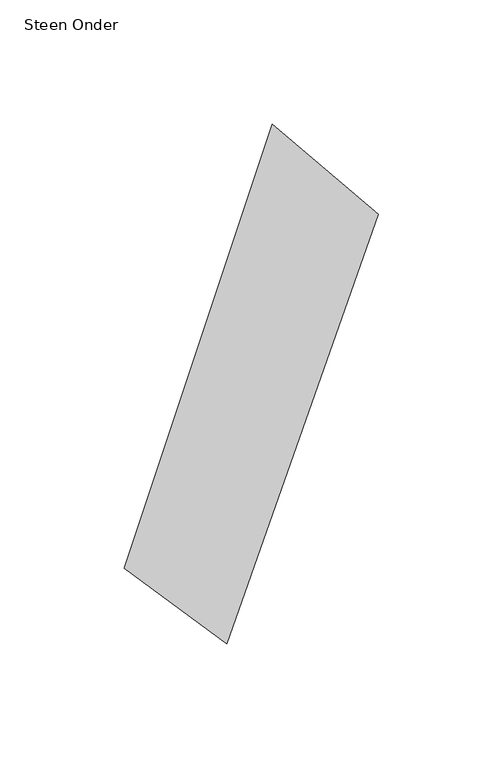
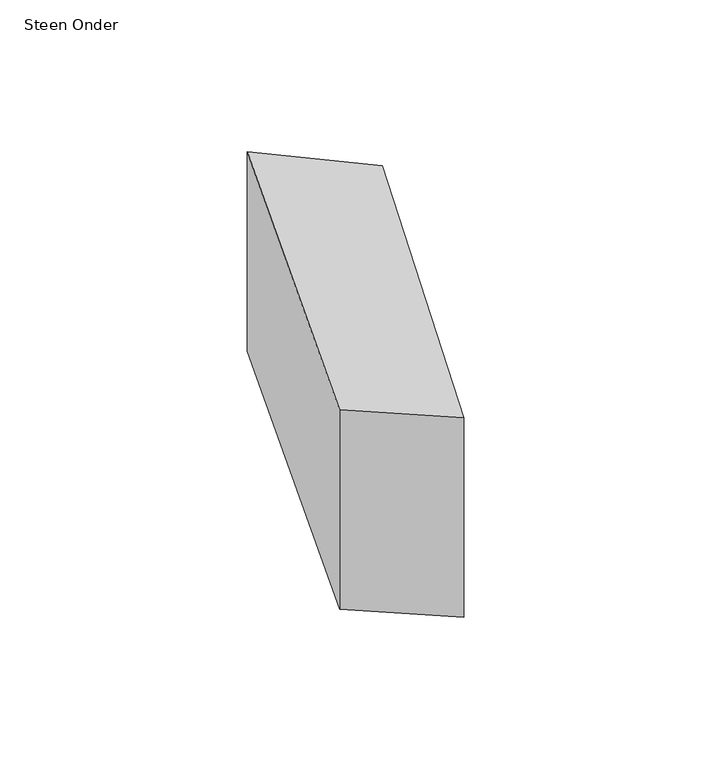
"""IFC4 building model written with IfcOpenShell, lengths in millimetres: proxy geometry, 00_GMA_steen_versie_4 : Steen Onder."""

from ifc_helpers import new_model, si_unit, origin, origin_with_axes, place, context, project, spatial, polyline, outline, extrude, source, transform, mapped, element, save


def steen_onder_4a2deff1(model_context):
    return source(origin(), model_context, "Body", "SweptSolid", [
        extrude(outline(polyline([(131.3416935, 155.8561718), (70.3187, -17.1071988), (28.9733706, 13.2506702), (88.516684, 192.1403058), (131.3416935, 155.8561718)])), origin_with_axes(), (0.0, 0.0, 1.0), 100.0),
    ])


if __name__ == "__main__":
    model = new_model("IFC4")
    model_context = context("Model", 3, world=origin())
    ifc_project = project(units=[si_unit("LENGTHUNIT", "METRE", prefix="MILLI")], contexts=[model_context])
    site = spatial("IfcSite", under=ifc_project)
    building = spatial("IfcBuilding", under=site)
    placement = place(None, origin())
    steen_onder_shape = steen_onder_4a2deff1(model_context)
    element("IfcBuildingElementProxy", 1, Name="00_GMA_steen_versie_4 : Steen Onder", ObjectType="00_GMA_steen_versie_4 : Steen Onder", at=placement, inside=building, context=model_context, shape_type="MappedRepresentation", body=[
        mapped(steen_onder_shape, transform((0.0, 0.0, 0.0), x_axis=(1.0, 0.0, 0.0), y_axis=(0.0, 1.0, 0.0), z_axis=(0.0, 0.0, 1.0))),
    ])
    save(model, "model.ifc")

# Revit data of these elements
# Type "00_GMA_steen_versie_4 : Steen Onder"
#   StootVoegHalfBoven [instance default] = 5 mm
#   StootVoegHalf [instance default] = 5 mm
#   StootVoegBreedteOnder = 10 mm
#   StootVoegBreedteBoven = 10 mm
#   Steendikte = 100 mm
#   LintVoegOnderHalf = 0 mm
#   LintVoegOnder = 0 mm
#   LintVoegBovenHalf = 5 mm
#   LintVoegBoven = 10 mm
#   materiaal = none
#   MateriaalVoeg = none
#   Default Elevation = 0
